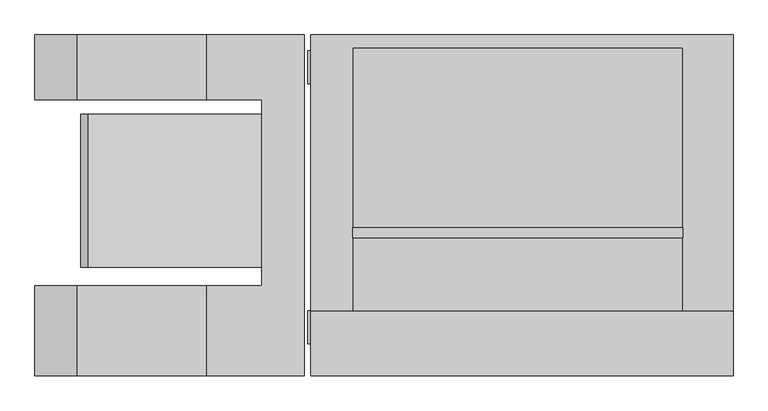
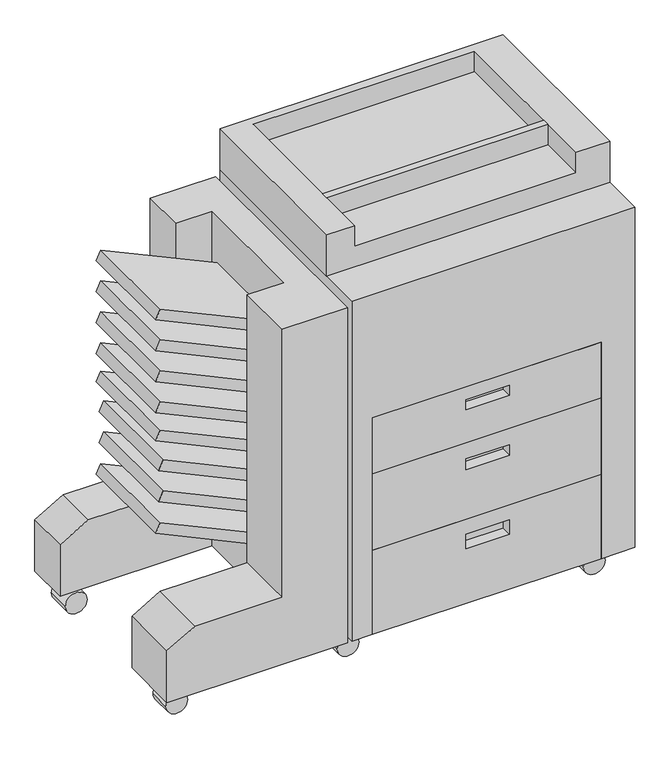
"""IFC4 building model written with IfcOpenShell, lengths in millimetres: proxy geometry, Kopierer : Kopierer."""

from ifc_helpers import new_model, si_unit, point, frame, frame_2d, origin, place, context, project, spatial, polyline, circle_curve, trimmed, segment, composite_curve, outline, extrude, faceted_brep, source, transform, mapped, element, save


def specialty_equipment_2d14421c(model_context):
    return source(origin(), model_context, "Body", "SolidModel", [
        extrude(outline(polyline([(387.7567294, -681.6535349), (364.7365116, -692.3880388), (232.9041289, -409.6725817), (260.929928, -409.6725817), (387.7567294, -681.6535349)])), frame((0.0, -72.1685532, 0.0), z_axis=(0.0, 1.0, 0.0), x_axis=(0.0, 0.0, 1.0)), (0.0, 0.0, 1.0), 239.8222339),
        extrude(outline(polyline([(463.6667654, -675.0122673), (440.6465476, -685.7467712), (311.9110388, -409.6725817), (339.9368379, -409.6725817), (463.6667654, -675.0122673)])), frame((0.0, -72.1685532, 0.0), z_axis=(0.0, 1.0, 0.0), x_axis=(0.0, 0.0, 1.0)), (0.0, 0.0, 1.0), 239.8222339),
        extrude(outline(polyline([(539.8667654, -675.0122673), (516.8465476, -685.7467712), (388.1110388, -409.6725817), (416.1368379, -409.6725817), (539.8667654, -675.0122673)])), frame((0.0, -72.1685532, 0.0), z_axis=(0.0, 1.0, 0.0), x_axis=(0.0, 0.0, 1.0)), (0.0, 0.0, 1.0), 239.8222339),
        extrude(outline(polyline([(914.2268014, -681.6535349), (891.2065836, -692.3880388), (759.3742009, -409.6725817), (787.4, -409.6725817), (914.2268014, -681.6535349)])), frame((0.0, -72.1685532, 0.0), z_axis=(0.0, 1.0, 0.0), x_axis=(0.0, 0.0, 1.0)), (0.0, 0.0, 1.0), 239.8222339),
        extrude(outline(polyline([(838.0268014, -681.6535349), (815.0065836, -692.3880388), (683.1742009, -409.6725817), (711.2, -409.6725817), (838.0268014, -681.6535349)])), frame((0.0, -72.1685532, 0.0), z_axis=(0.0, 1.0, 0.0), x_axis=(0.0, 0.0, 1.0)), (0.0, 0.0, 1.0), 239.8222339),
        extrude(outline(polyline([(615.7768014, -681.6535349), (592.7565836, -692.3880388), (460.9242009, -409.6725817), (488.95, -409.6725817), (615.7768014, -681.6535349)])), frame((0.0, -72.1685532, 0.0), z_axis=(0.0, 1.0, 0.0), x_axis=(0.0, 0.0, 1.0)), (0.0, 0.0, 1.0), 239.8222339),
        extrude(outline(polyline([(685.6268014, -681.6535349), (662.6065836, -692.3880388), (530.7742009, -409.6725817), (558.8, -409.6725817), (685.6268014, -681.6535349)])), frame((0.0, -72.1685532, 0.0), z_axis=(0.0, 1.0, 0.0), x_axis=(0.0, 0.0, 1.0)), (0.0, 0.0, 1.0), 239.8222339),
        extrude(outline(polyline([(761.8268014, -681.6535349), (738.8065836, -692.3880388), (606.9742009, -409.6725817), (635.0, -409.6725817), (761.8268014, -681.6535349)])), frame((0.0, -72.1685532, 0.0), z_axis=(0.0, 1.0, 0.0), x_axis=(0.0, 0.0, 1.0)), (0.0, 0.0, 1.0), 239.8222339),
        extrude(outline(composite_curve([segment(trimmed(circle_curve(frame_2d((26.0668925, -711.8709821)), 25.4), [point((26.0668925, -737.2709821))], [point((26.0668925, -686.4709821))], False, "CARTESIAN"), True, "CONTINUOUS"), segment(trimmed(circle_curve(frame_2d((26.0668925, -711.8709821)), 25.4), [point((26.0668925, -686.4709821))], [point((26.0668925, -737.2709821))], False, "CARTESIAN"), True, "CONTINUOUS")], self_intersect=False)), frame((0.0, 215.1689468, 0.0), z_axis=(0.0, 1.0, 0.0), x_axis=(0.0, 0.0, 1.0)), (0.0, 0.0, 1.0), 55.9418879),
        extrude(outline(composite_curve([segment(trimmed(circle_curve(frame_2d((26.0668925, -711.8709821)), 25.4), [point((26.0668925, -737.2709821))], [point((26.0668925, -686.4709821))], False, "CARTESIAN"), True, "CONTINUOUS"), segment(trimmed(circle_curve(frame_2d((26.0668925, -711.8709821)), 25.4), [point((26.0668925, -686.4709821))], [point((26.0668925, -737.2709821))], False, "CARTESIAN"), True, "CONTINUOUS")], self_intersect=False)), frame((0.0, -191.2310532, 0.0), z_axis=(0.0, 1.0, 0.0), x_axis=(0.0, 0.0, 1.0)), (0.0, 0.0, 1.0), 51.3258053),
        faceted_brep([(-764.1654582, -242.0310532, 76.2), (-342.5743224, -242.0310532, 76.2), (-342.5743224, -242.0310532, 901.7), (-494.9743224, -242.0310532, 901.7), (-494.9743224, -242.0310532, 241.3), (-698.1743224, -242.0310532, 241.3), (-764.1654582, -242.0310532, 203.2), (-764.1654582, 291.3689468, 76.2), (-764.1654582, 291.3689468, 203.2), (-698.1743224, 291.3689468, 241.3), (-494.9743224, 291.3689468, 241.3), (-494.9743224, 291.3689468, 901.7), (-342.5743224, 291.3689468, 901.7), (-342.5743224, 291.3689468, 76.2), (-764.1654582, -100.8888364, 76.2), (-409.6725817, -100.8888364, 76.2), (-409.6725817, 189.7689468, 76.2), (-764.1654582, 189.7689468, 76.2), (-494.9743224, 189.7689468, 901.7), (-409.6725817, 189.7689468, 901.7), (-409.6725817, -100.8888364, 901.7), (-494.9743224, -100.8888364, 901.7), (-494.9743224, -100.8888364, 241.3), (-494.9743224, 189.7689468, 241.3), (-698.1743224, -100.8888364, 241.3), (-698.1743224, 189.7689468, 241.3), (-764.1654582, -100.8888364, 203.2), (-764.1654582, 189.7689468, 203.2)], [[[0, 1, 2, 3, 4, 5, 6]], [[7, 8, 9, 10, 11, 12, 13]], [[1, 0, 14, 15, 16, 17, 7, 13]], [[2, 1, 13, 12]], [[3, 2, 12, 11, 18, 19, 20, 21]], [[4, 3, 21, 22]], [[11, 10, 23, 18]], [[5, 4, 22, 24]], [[10, 9, 25, 23]], [[6, 5, 24, 26]], [[9, 8, 27, 25]], [[0, 6, 26, 14]], [[8, 7, 17, 27]], [[16, 19, 18, 23, 25, 27, 17]], [[20, 15, 14, 26, 24, 22, 21]], [[19, 16, 15, 20]]]),
        extrude(outline(composite_curve([segment(trimmed(circle_curve(frame_2d((27.9129458, -312.2555429)), 25.4), [point((27.9129458, -337.6555429))], [point((27.9129458, -286.8555429))], False, "CARTESIAN"), True, "CONTINUOUS"), segment(trimmed(circle_curve(frame_2d((27.9129458, -312.2555429)), 25.4), [point((27.9129458, -286.8555429))], [point((27.9129458, -337.6555429))], False, "CARTESIAN"), True, "CONTINUOUS")], self_intersect=False)), frame((0.0, 215.1689468, 0.0), z_axis=(0.0, 1.0, 0.0), x_axis=(0.0, 0.0, 1.0)), (0.0, 0.0, 1.0), 51.3258053),
        extrude(outline(composite_curve([segment(trimmed(circle_curve(frame_2d((27.9129458, 262.7398948)), 25.4), [point((27.9129458, 237.3398948))], [point((27.9129458, 288.1398948))], False, "CARTESIAN"), True, "CONTINUOUS"), segment(trimmed(circle_curve(frame_2d((27.9129458, 262.7398948)), 25.4), [point((27.9129458, 288.1398948))], [point((27.9129458, 237.3398948))], False, "CARTESIAN"), True, "CONTINUOUS")], self_intersect=False)), frame((0.0, 215.1689468, 0.0), z_axis=(0.0, 1.0, 0.0), x_axis=(0.0, 0.0, 1.0)), (0.0, 0.0, 1.0), 51.3258053),
        extrude(outline(composite_curve([segment(trimmed(circle_curve(frame_2d((27.9129458, -312.2555429)), 25.4), [point((27.9129458, -337.6555429))], [point((27.9129458, -286.8555429))], False, "CARTESIAN"), True, "CONTINUOUS"), segment(trimmed(circle_curve(frame_2d((27.9129458, -312.2555429)), 25.4), [point((27.9129458, -286.8555429))], [point((27.9129458, -337.6555429))], False, "CARTESIAN"), True, "CONTINUOUS")], self_intersect=False)), frame((0.0, -191.2310532, 0.0), z_axis=(0.0, 1.0, 0.0), x_axis=(0.0, 0.0, 1.0)), (0.0, 0.0, 1.0), 51.3258053),
        extrude(outline(composite_curve([segment(trimmed(circle_curve(frame_2d((27.9129458, 262.7398948)), 25.4), [point((27.9129458, 237.3398948))], [point((27.9129458, 288.1398948))], False, "CARTESIAN"), True, "CONTINUOUS"), segment(trimmed(circle_curve(frame_2d((27.9129458, 262.7398948)), 25.4), [point((27.9129458, 288.1398948))], [point((27.9129458, 237.3398948))], False, "CARTESIAN"), True, "CONTINUOUS")], self_intersect=False)), frame((0.0, -191.2310532, 0.0), z_axis=(0.0, 1.0, 0.0), x_axis=(0.0, 0.0, 1.0)), (0.0, 0.0, 1.0), 51.3258053),
        extrude(outline(polyline([(249.314028, -26.1310532), (-267.2959958, -26.1310532), (-267.2959958, -10.0577181), (249.314028, -10.0577181), (249.314028, -26.1310532)])), frame((0.0, 0.0, 965.2), z_axis=(0.0, 0.0, 1.0), x_axis=(1.0, 0.0, 0.0)), (0.0, 0.0, 1.0), 50.8),
        faceted_brep([(249.314028, -242.0310532, 472.3553727), (249.314028, -242.0310532, 609.6), (-284.085972, -242.0310532, 609.6), (-284.085972, -242.0310532, 472.3553727), (-66.7741493, -242.0310532, 578.8591447), (34.8258507, -242.0310532, 578.8591447), (34.8258507, -242.0310532, 553.4591447), (-66.7741493, -242.0310532, 553.4591447), (249.314028, -191.2310532, 472.3553727), (-284.085972, -191.2310532, 472.3553727), (-284.085972, -191.2310532, 609.6), (249.314028, -191.2310532, 609.6), (34.8258507, -216.6310532, 578.8591447), (-66.7741493, -216.6310532, 578.8591447), (-66.7741493, -216.6310532, 553.4591447), (34.8258507, -216.6310532, 553.4591447)], [[[0, 1, 2, 3], [4, 5, 6, 7]], [[8, 9, 10, 11]], [[1, 0, 8, 11]], [[2, 1, 11, 10]], [[3, 2, 10, 9]], [[0, 3, 9, 8]], [[12, 13, 14, 15]], [[13, 12, 5, 4]], [[14, 13, 4, 7]], [[15, 14, 7, 6]], [[12, 15, 6, 5]]]),
        faceted_brep([(249.314028, -242.0310532, 283.8723489), (249.314028, -242.0310532, 472.3553727), (-284.085972, -242.0310532, 472.3553727), (-284.085972, -242.0310532, 283.8723489), (-66.7741493, -242.0310532, 432.3774172), (34.8258507, -242.0310532, 432.3774172), (34.8258507, -242.0310532, 406.4), (-66.7741493, -242.0310532, 406.4), (249.314028, -191.2310532, 283.8723489), (-284.085972, -191.2310532, 283.8723489), (-284.085972, -191.2310532, 472.3553727), (249.314028, -191.2310532, 472.3553727), (34.8258507, -216.6310532, 432.3774172), (-66.7741493, -216.6310532, 432.3774172), (-66.7741493, -216.6310532, 406.4), (34.8258507, -216.6310532, 406.4)], [[[0, 1, 2, 3], [4, 5, 6, 7]], [[8, 9, 10, 11]], [[1, 0, 8, 11]], [[2, 1, 11, 10]], [[3, 2, 10, 9]], [[0, 3, 9, 8]], [[12, 13, 14, 15]], [[13, 12, 5, 4]], [[14, 13, 4, 7]], [[15, 14, 7, 6]], [[12, 15, 6, 5]]]),
        faceted_brep([(249.314028, -242.0310532, 76.2), (249.314028, -242.0310532, 283.8723489), (-284.085972, -242.0310532, 283.8723489), (-284.085972, -242.0310532, 76.2), (-66.7741493, -242.0310532, 246.5423898), (34.8258507, -242.0310532, 246.5423898), (34.8258507, -242.0310532, 211.1096445), (-66.7741493, -242.0310532, 211.1096445), (249.314028, -191.2310532, 76.2), (-284.085972, -191.2310532, 76.2), (-284.085972, -191.2310532, 283.8723489), (249.314028, -191.2310532, 283.8723489), (34.8258507, -216.6310532, 246.5423898), (-66.7741493, -216.6310532, 246.5423898), (-66.7741493, -216.6310532, 211.1096445), (34.8258507, -216.6310532, 211.1096445)], [[[0, 1, 2, 3], [4, 5, 6, 7]], [[8, 9, 10, 11]], [[1, 0, 8, 11]], [[2, 1, 11, 10]], [[3, 2, 10, 9]], [[0, 3, 9, 8]], [[12, 13, 14, 15]], [[13, 12, 5, 4]], [[14, 13, 4, 7]], [[15, 14, 7, 6]], [[12, 15, 6, 5]]]),
        faceted_brep([(328.0345418, 291.3689468, 1016.0), (-332.3654582, 291.3689468, 1016.0), (-332.3654582, -139.9052479, 1016.0), (-267.2959958, -139.9052479, 1016.0), (-267.2959958, 271.1108348, 1016.0), (249.314028, 271.1108348, 1016.0), (249.314028, -139.9052479, 1016.0), (328.0345418, -139.9052479, 1016.0), (328.0345418, 291.3689468, 914.4), (328.0345418, -139.9052479, 914.4), (-332.3654582, -139.9052479, 914.4), (-332.3654582, 291.3689468, 914.4), (249.314028, -139.9052479, 965.2), (-267.2959958, -139.9052479, 965.2), (249.314028, 271.1108348, 965.2), (-267.2959958, 271.1108348, 965.2)], [[[0, 1, 2, 3, 4, 5, 6, 7]], [[8, 9, 10, 11]], [[1, 0, 8, 11]], [[2, 1, 11, 10]], [[10, 9, 7, 6, 12, 13, 3, 2]], [[0, 7, 9, 8]], [[14, 15, 13, 12]], [[15, 14, 5, 4]], [[13, 15, 4, 3]], [[14, 12, 6, 5]]]),
        faceted_brep([(328.0345418, 291.3689468, 914.4), (-332.3654582, 291.3689468, 914.4), (-332.3654582, -242.0310532, 914.4), (328.0345418, -242.0310532, 914.4), (328.0345418, 291.3689468, 76.2), (328.0345418, -242.0310532, 76.2), (249.314028, -242.0310532, 76.2), (249.314028, -191.2310532, 76.2), (-284.085972, -191.2310532, 76.2), (-284.085972, -242.0310532, 76.2), (-332.3654582, -242.0310532, 76.2), (-332.3654582, 291.3689468, 76.2), (-284.085972, -242.0310532, 609.6), (249.314028, -242.0310532, 609.6), (-284.085972, -191.2310532, 609.6), (249.314028, -191.2310532, 609.6)], [[[0, 1, 2, 3]], [[4, 5, 6, 7, 8, 9, 10, 11]], [[1, 0, 4, 11]], [[2, 1, 11, 10]], [[3, 2, 10, 9, 12, 13, 6, 5]], [[0, 3, 5, 4]], [[14, 8, 7, 15]], [[8, 14, 12, 9]], [[15, 7, 6, 13]], [[14, 15, 13, 12]]]),
    ])


if __name__ == "__main__":
    model = new_model("IFC4")
    model_context = context("Model", 3, world=origin())
    ifc_project = project(units=[si_unit("LENGTHUNIT", "METRE", prefix="MILLI")], contexts=[model_context])
    site = spatial("IfcSite", under=ifc_project)
    building = spatial("IfcBuilding", under=site)
    placement = place(None, origin())
    specialty_equipment_shape = specialty_equipment_2d14421c(model_context)
    element("IfcBuildingElementProxy", 1, Name="Kopierer : Kopierer", ObjectType="Kopierer : Kopierer", at=placement, inside=building, context=model_context, shape_type="MappedRepresentation", body=[
        mapped(specialty_equipment_shape, transform((0.0, 0.0, 0.0), x_axis=(1.0, 0.0, 0.0), y_axis=(0.0, 1.0, 0.0), z_axis=(0.0, 0.0, 1.0))),
    ])
    save(model, "model.ifc")

# Revit data of these elements
# Type "Kopierer : Kopierer"
#   Assembly Code = ""
# Element 1 (IfcBuildingElementProxy, "Kopierer : Kopierer")
#   Materials on its faces: "Kunststoff - Weiß", "Kunststoff - grau, dunkel"
# Materials
#   "Kunststoff - Weiß": class "Kunststoff", colour RGB 249 249 249, transparency 0, Cost = 0
#   "Kunststoff - grau, dunkel": class "Kunststoff", colour RGB 134 134 134, transparency 0
